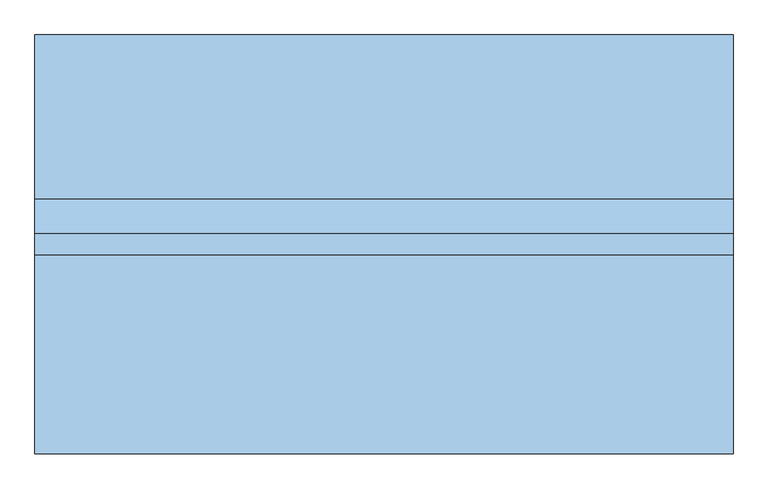
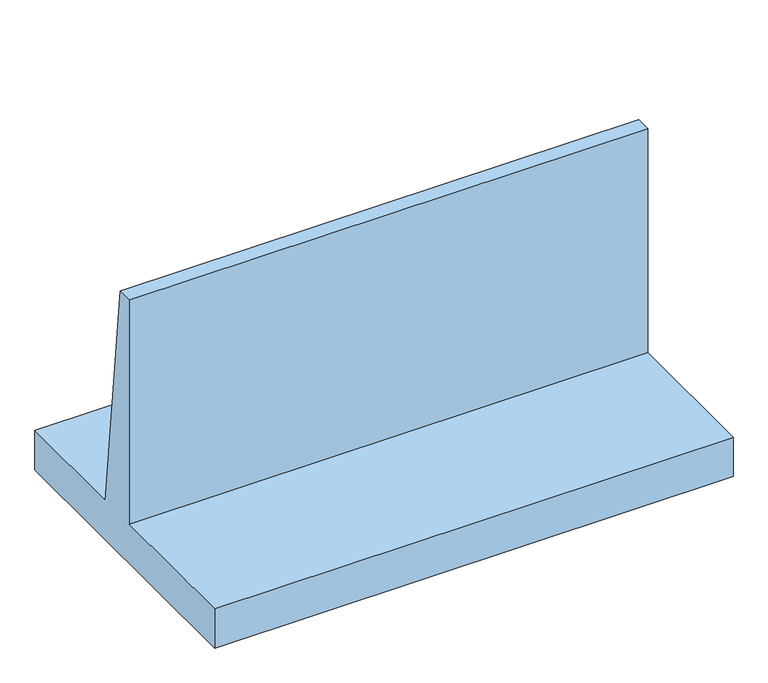
"""IFC4 building model written with IfcOpenShell, lengths in millimetres: window geometry, RTAINING_WALL : RTAINING_WALL."""

from ifc_helpers import new_model, si_unit, frame, origin, place, context, project, spatial, polyline, outline, extrude, source, transform, mapped, element, save


def window_4402a012(model_context):
    return source(origin(), model_context, "Body", "SweptSolid", [
        extrude(outline(polyline([(5260.6690419, -2500.0), (5260.6690419, 2072.0), (5560.6690419, 2072.0), (6060.6690419, -2500.0), (8410.6690419, -2500.0), (8410.6690419, -3300.0), (2410.6690419, -3300.0), (2410.6690419, -2500.0), (5260.6690419, -2500.0)])), frame((-12426.8014101, 0.0, 0.0), z_axis=(1.0, 0.0, 0.0), x_axis=(0.0, 1.0, 0.0)), (0.0, 0.0, 1.0), 10000.0),
    ])


if __name__ == "__main__":
    model = new_model("IFC4")
    model_context = context("Model", 3, world=origin())
    ifc_project = project(units=[si_unit("LENGTHUNIT", "METRE", prefix="MILLI")], contexts=[model_context])
    site = spatial("IfcSite", under=ifc_project)
    building = spatial("IfcBuilding", under=site)
    placement = place(None, origin())
    window_shape = window_4402a012(model_context)
    element("IfcWindow", 1, ObjectType="RTAINING_WALL : RTAINING_WALL", at=placement, inside=building, context=model_context, shape_type="MappedRepresentation", body=[
        mapped(window_shape, transform((0.0, 0.0, 0.0), x_axis=(1.0, 0.0, 0.0), y_axis=(0.0, 1.0, 0.0), z_axis=(0.0, 0.0, 1.0))),
    ])
    save(model, "model.ifc")

# Revit data of these elements
# Project information
#   Project Issue Date = "Issue Date"
#   Project Status = "Project Status"
#   Client Name = "Owner"
#   Project Address = "Enter address here"
#   Project Name = "Project Name"
#   Project Number = "0001"
# Type "RTAINING_WALL : RTAINING_WALL"
#   Type Mark = "27"
# Element 1 (IfcWindow, "RTAINING_WALL : RTAINING_WALL")
#   Materials on its faces: "Concrete, Cast In Situ"
# Materials
#   "Concrete, Cast In Situ": class "Concrete", colour RGB 192 192 192, transparency 0, Description = "physical material", Cost = 0
